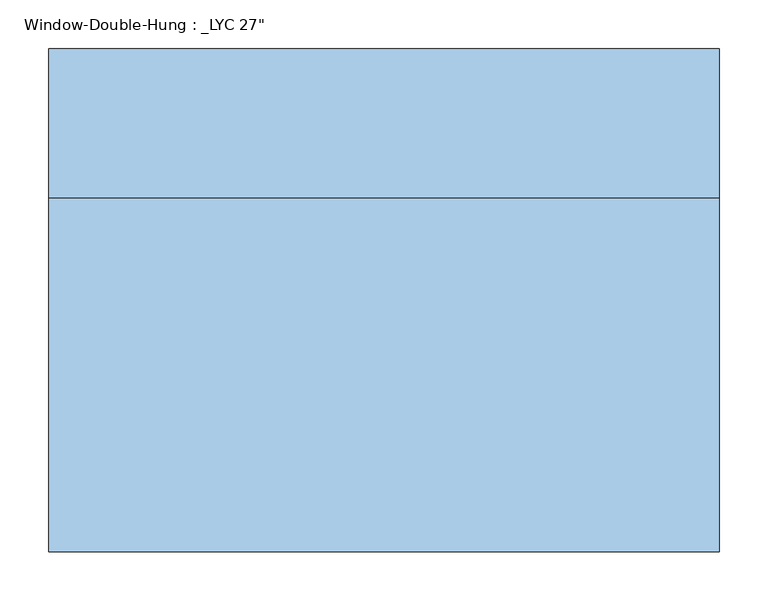
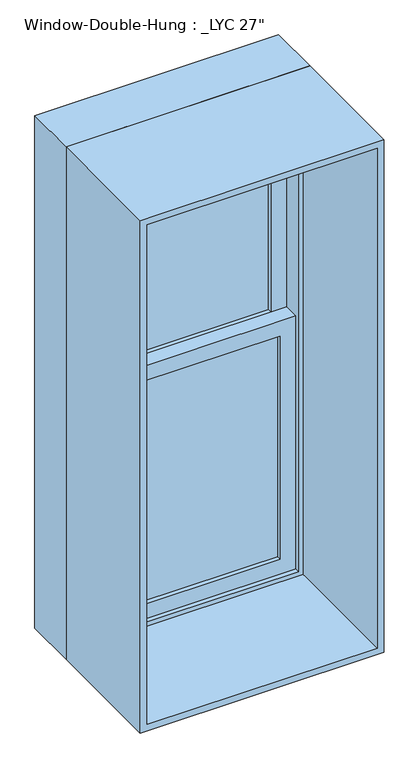
"""IFC4 building model written with IfcOpenShell, lengths in millimetres: window geometry."""

from ifc_helpers import new_model, si_unit, frame, origin, place, context, project, spatial, polyline, outline, extrude, source, transform, mapped, element, save


def window_acb6bd2b(model_context):
    return source(origin(), model_context, "Body", "SweptSolid", [
        extrude(outline(polyline([(266.7, 158.75), (266.7, 152.4), (-266.7, 152.4), (-266.7, 158.75), (266.7, 158.75)])), frame((0.0, 0.0, 990.6), z_axis=(0.0, 0.0, 1.0), x_axis=(1.0, 0.0, 0.0)), (0.0, 0.0, 1.0), 663.575),
        extrude(outline(polyline([(-266.7, 146.05), (266.7, 146.05), (266.7, 139.7), (-266.7, 139.7), (-266.7, 146.05)])), frame((0.0, 0.0, 990.6), z_axis=(0.0, 0.0, 1.0), x_axis=(1.0, 0.0, 0.0)), (0.0, 0.0, 1.0), 663.575),
        extrude(outline(polyline([(266.7, 203.2), (266.7, 196.85), (-266.7, 196.85), (-266.7, 203.2), (266.7, 203.2)])), frame((0.0, 0.0, 1698.625), z_axis=(0.0, 0.0, 1.0), x_axis=(1.0, 0.0, 0.0)), (0.0, 0.0, 1.0), 663.575),
        extrude(outline(polyline([(-266.7, 190.5), (266.7, 190.5), (266.7, 184.15), (-266.7, 184.15), (-266.7, 190.5)])), frame((0.0, 0.0, 1698.625), z_axis=(0.0, 0.0, 1.0), x_axis=(1.0, 0.0, 0.0)), (0.0, 0.0, 1.0), 663.575),
        extrude(outline(polyline([(1698.625, -311.15), (946.15, -311.15), (946.15, 311.15), (1698.625, 311.15), (1698.625, -311.15)]), holes=[polyline([(1654.175, 266.7), (990.6, 266.7), (990.6, -266.7), (1654.175, -266.7), (1654.175, 266.7)])]), frame((0.0, 127.0, 0.0), z_axis=(0.0, 1.0, 0.0), x_axis=(0.0, 0.0, 1.0)), (0.0, 0.0, 1.0), 44.45),
        extrude(outline(polyline([(2406.65, -311.15), (1654.175, -311.15), (1654.175, 311.15), (2406.65, 311.15), (2406.65, -311.15)]), holes=[polyline([(2362.2, 266.7), (1698.625, 266.7), (1698.625, -266.7), (2362.2, -266.7), (2362.2, 266.7)])]), frame((0.0, 171.45, 0.0), z_axis=(0.0, 1.0, 0.0), x_axis=(0.0, 0.0, 1.0)), (0.0, 0.0, 1.0), 44.45),
        extrude(outline(polyline([(2438.4, -342.9), (914.4, -342.9), (914.4, 342.9), (2438.4, 342.9), (2438.4, -342.9)]), holes=[polyline([(2406.65, 311.15), (946.15, 311.15), (946.15, -311.15), (2406.65, -311.15), (2406.65, 311.15)])]), frame((0.0, 114.3, 0.0), z_axis=(0.0, 1.0, 0.0), x_axis=(0.0, 0.0, 1.0)), (0.0, 0.0, 1.0), 152.4),
        extrude(outline(polyline([(2438.4, 342.9), (2438.4, -342.9), (914.4, -342.9), (914.4, 342.9), (2438.4, 342.9)]), holes=[polyline([(2419.35, 323.85), (933.45, 323.85), (933.45, -323.85), (2419.35, -323.85), (2419.35, 323.85)])]), frame((0.0, -247.65, 0.0), z_axis=(0.0, 1.0, 0.0), x_axis=(0.0, 0.0, 1.0)), (0.0, 0.0, 1.0), 361.95),
    ])


if __name__ == "__main__":
    model = new_model("IFC4")
    model_context = context("Model", 3, world=origin())
    ifc_project = project(units=[si_unit("LENGTHUNIT", "METRE", prefix="MILLI")], contexts=[model_context])
    site = spatial("IfcSite", under=ifc_project)
    building = spatial("IfcBuilding", under=site)
    placement = place(None, origin())
    window_shape = window_acb6bd2b(model_context)
    element("IfcWindow", 1, ObjectType="Window-Double-Hung : _LYC 27\"", at=placement, inside=building, context=model_context, shape_type="MappedRepresentation", body=[
        mapped(window_shape, transform((0.0, 0.0, 0.0), x_axis=(1.0, 0.0, 0.0), y_axis=(0.0, 1.0, 0.0), z_axis=(0.0, 0.0, 1.0))),
    ])
    save(model, "model.ifc")

# Revit data of these elements
# Type "Window-Double-Hung : _LYC 27\""
#   Type Mark = "24"
#   Fire Rating = "0.5h"
#   Assembly Code = "B2020100"
#   Wall Thickness [instance default] = 0' - 6"
#   Visual Light Transmittance = 0.9
#   Thermal Resistance (R) = 1.8146 (h·ft²·°F)/BTU
#   Solar Heat Gain Coefficient = 0.78
#   Rough Width = 2' - 3 1/2"
#   Rough Height = 5' - 0 1/2"
#   Muntin Width = 1' - 9"
#   Muntin Height = 2' - 2 1/8"
#   Interior Wall Closure [instance default] = 0' - 1 1/2"
#   Heat Transfer Coefficient (U) = 0.6496 BTU/(h·ft²·°F)
#   Frame Extension [instance default] = 0' - 2"
#   Exterior Wall Closure [instance default] = 0' - 0 1/2"
#   Extension Jamb [instance default] = 0' - 0 3/4"
#   Height = 5' - 0"
#   Width = 2' - 3"
#   Window Inset [instance default] = 0' - 0 3/4"
#   Top Muntin Visibility = yes
#   Interior Trim Visibility [instance default] = yes
#   Indicator Visibility [instance default] = yes
#   Exterior Trim Visibility [instance default] = yes
#   Extension Jamb Visibility [instance default] = yes
#   Define Thermal Properties by = 1
#   Bottom Muntin Visibility = yes
#   Muntin Pattern = Muntin Pattern_2x2 : Muntin Pattern_2x2
#   Interior Trim Material = Wood - Stained
#   Interior Trim = Trim-Window-Interior-Flat : Picture Frame
#   Interior Frame Material = Wood - Stained
#   Glass Panel Material = Glass
#   Exterior Trim Material = Clad - White
#   Exterior Trim = Trim-Window-Exterior-Flat : with Sill
#   Exterior Frame Material = Clad - White
#   Construction Type Id = ""
#   Wall Closure = (empty or 0)
#   Analytic Construction = (empty or 0)
# Element 1 (IfcWindow, "Window-Double-Hung : _LYC 27\"")
#   Wall Thickness = 1' - 7 1/2"
#   Extension Jamb = 1' - 2 1/4"
#   Materials on its faces: "Wood - Stained", "Glass", "Clad - White"
# Materials
#   "Wood - Stained": class "Wood", colour RGB 224 178 126, transparency 0, Cost = 0
#   "Glass": class "Unassigned", colour RGB 0 128 192, transparency 0.75
#   "Clad - White": class "Wood", colour RGB 242 242 238, transparency 0, Cost = 0
